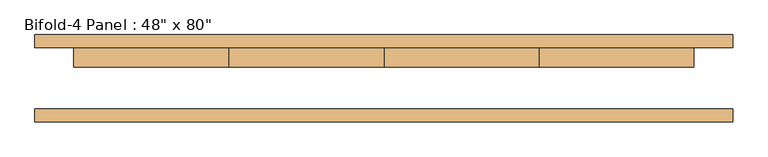
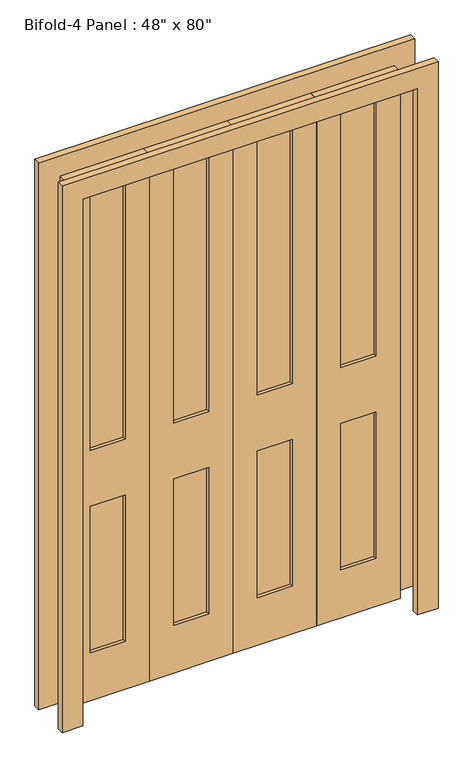
"""IFC4 building model written with IfcOpenShell, lengths in millimetres: door geometry."""

from ifc_helpers import new_model, si_unit, frame, origin, place, context, project, spatial, polyline, outline, extrude, source, transform, mapped, element, save


def door_5b0cfbe2(model_context):
    return source(origin(), model_context, "Body", "SweptSolid", [
        extrude(outline(polyline([(393.7, 47.625), (520.7, 47.625), (520.7, 34.925), (393.7, 34.925), (393.7, 47.625)])), frame((0.0, 0.0, 965.2), z_axis=(0.0, 0.0, 1.0), x_axis=(1.0, 0.0, 0.0)), (0.0, 0.0, 1.0), 984.25),
        extrude(outline(polyline([(393.7, 47.625), (520.7, 47.625), (520.7, 34.925), (393.7, 34.925), (393.7, 47.625)])), frame((0.0, 0.0, 184.15), z_axis=(0.0, 0.0, 1.0), x_axis=(1.0, 0.0, 0.0)), (0.0, 0.0, 1.0), 565.15),
        extrude(outline(polyline([(88.9, 47.625), (215.9, 47.625), (215.9, 34.925), (88.9, 34.925), (88.9, 47.625)])), frame((0.0, 0.0, 965.2), z_axis=(0.0, 0.0, 1.0), x_axis=(1.0, 0.0, 0.0)), (0.0, 0.0, 1.0), 984.25),
        extrude(outline(polyline([(88.9, 47.625), (215.9, 47.625), (215.9, 34.925), (88.9, 34.925), (88.9, 47.625)])), frame((0.0, 0.0, 184.15), z_axis=(0.0, 0.0, 1.0), x_axis=(1.0, 0.0, 0.0)), (0.0, 0.0, 1.0), 565.15),
        extrude(outline(polyline([(-215.9, 47.625), (-88.9, 47.625), (-88.9, 34.925), (-215.9, 34.925), (-215.9, 47.625)])), frame((0.0, 0.0, 184.15), z_axis=(0.0, 0.0, 1.0), x_axis=(1.0, 0.0, 0.0)), (0.0, 0.0, 1.0), 565.15),
        extrude(outline(polyline([(-215.9, 47.625), (-88.9, 47.625), (-88.9, 34.925), (-215.9, 34.925), (-215.9, 47.625)])), frame((0.0, 0.0, 965.2), z_axis=(0.0, 0.0, 1.0), x_axis=(1.0, 0.0, 0.0)), (0.0, 0.0, 1.0), 984.25),
        extrude(outline(polyline([(-520.7, 47.625), (-393.7, 47.625), (-393.7, 34.925), (-520.7, 34.925), (-520.7, 47.625)])), frame((0.0, 0.0, 965.2), z_axis=(0.0, 0.0, 1.0), x_axis=(1.0, 0.0, 0.0)), (0.0, 0.0, 1.0), 984.25),
        extrude(outline(polyline([(-520.7, 47.625), (-393.7, 47.625), (-393.7, 34.925), (-520.7, 34.925), (-520.7, 47.625)])), frame((0.0, 0.0, 184.15), z_axis=(0.0, 0.0, 1.0), x_axis=(1.0, 0.0, 0.0)), (0.0, 0.0, 1.0), 565.15),
        extrude(outline(polyline([(0.0, 685.8), (2108.2, 685.8), (2108.2, -685.8), (0.0, -685.8), (0.0, -609.6), (2032.0, -609.6), (2032.0, 609.6), (0.0, 609.6), (0.0, 685.8)])), frame((0.0, -85.725, 0.0), z_axis=(0.0, 1.0, 0.0), x_axis=(0.0, 0.0, 1.0)), (0.0, 0.0, 1.0), 25.4),
        extrude(outline(polyline([(0.0, 685.8), (2108.2, 685.8), (2108.2, -685.8), (0.0, -685.8), (0.0, -609.6), (2032.0, -609.6), (2032.0, 609.6), (0.0, 609.6), (0.0, 685.8)])), frame((0.0, 60.325, 0.0), z_axis=(0.0, 1.0, 0.0), x_axis=(0.0, 0.0, 1.0)), (0.0, 0.0, 1.0), 25.4),
        extrude(outline(polyline([(0.0, -609.6), (0.0, -304.8), (2032.0, -304.8), (2032.0, -609.6), (0.0, -609.6)]), holes=[polyline([(1949.45, -520.7), (1949.45, -393.7), (965.2, -393.7), (965.2, -520.7), (1949.45, -520.7)]), polyline([(749.3, -520.7), (749.3, -393.7), (184.15, -393.7), (184.15, -520.7), (749.3, -520.7)])]), frame((0.0, 22.225, 0.0), z_axis=(0.0, 1.0, 0.0), x_axis=(0.0, 0.0, 1.0)), (0.0, 0.0, 1.0), 38.1),
        extrude(outline(polyline([(0.0, -304.8), (0.0, 0.0), (2032.0, 0.0), (2032.0, -304.8), (0.0, -304.8)]), holes=[polyline([(1949.45, -215.9), (1949.45, -88.9), (965.2, -88.9), (965.2, -215.9), (1949.45, -215.9)]), polyline([(749.3, -215.9), (749.3, -88.9), (184.15, -88.9), (184.15, -215.9), (749.3, -215.9)])]), frame((0.0, 22.225, 0.0), z_axis=(0.0, 1.0, 0.0), x_axis=(0.0, 0.0, 1.0)), (0.0, 0.0, 1.0), 38.1),
        extrude(outline(polyline([(0.0, 0.0), (0.0, 304.8), (2032.0, 304.8), (2032.0, 0.0), (0.0, 0.0)]), holes=[polyline([(1949.45, 88.9), (1949.45, 215.9), (965.2, 215.9), (965.2, 88.9), (1949.45, 88.9)]), polyline([(749.3, 88.9), (749.3, 215.9), (184.15, 215.9), (184.15, 88.9), (749.3, 88.9)])]), frame((0.0, 22.225, 0.0), z_axis=(0.0, 1.0, 0.0), x_axis=(0.0, 0.0, 1.0)), (0.0, 0.0, 1.0), 38.1),
        extrude(outline(polyline([(0.0, 304.8), (0.0, 609.6), (2032.0, 609.6), (2032.0, 304.8), (0.0, 304.8)]), holes=[polyline([(1949.45, 393.7), (1949.45, 520.7), (965.2, 520.7), (965.2, 393.7), (1949.45, 393.7)]), polyline([(749.3, 393.7), (749.3, 520.7), (184.15, 520.7), (184.15, 393.7), (749.3, 393.7)])]), frame((0.0, 22.225, 0.0), z_axis=(0.0, 1.0, 0.0), x_axis=(0.0, 0.0, 1.0)), (0.0, 0.0, 1.0), 38.1),
    ])


if __name__ == "__main__":
    model = new_model("IFC4")
    model_context = context("Model", 3, world=origin())
    ifc_project = project(units=[si_unit("LENGTHUNIT", "METRE", prefix="MILLI")], contexts=[model_context])
    site = spatial("IfcSite", under=ifc_project)
    building = spatial("IfcBuilding", under=site)
    placement = place(None, origin())
    door_shape = door_5b0cfbe2(model_context)
    element("IfcDoor", 1, ObjectType="Bifold-4 Panel : 48\" x 80\"", at=placement, inside=building, context=model_context, shape_type="MappedRepresentation", body=[
        mapped(door_shape, transform((0.0, 0.0, 0.0), x_axis=(1.0, 0.0, 0.0), y_axis=(0.0, 1.0, 0.0), z_axis=(0.0, 0.0, 1.0))),
    ])
    save(model, "model.ifc")

# Revit data of these elements
# Type "Bifold-4 Panel : 48\" x 80\""
#   Type Mark = "D9"
#   Assembly Code = "C1020"
#   Thickness = 0' - 1 1/2"
#   Height = 6' - 8"
#   Trim Width = 0' - 3"
#   Width = 4' - 0"
#   Door Material = Door - Panel
#   Frame Material = Door - Frame
#   Function = (empty or 0)
#   Description = (empty or 0)
#   Wall Closure = (empty or 0)
# Element 1 (IfcDoor, "Bifold-4 Panel : 48\" x 80\"")
#   Materials on its faces: "Door - Panel", "Door - Frame"
# Materials
#   "Door - Panel": class "Wood", colour RGB 210 159 95, transparency 0, Cost = 0
#   "Door - Frame": class "Miscellaneous", colour RGB 118 70 51, transparency 0, Cost = 0
